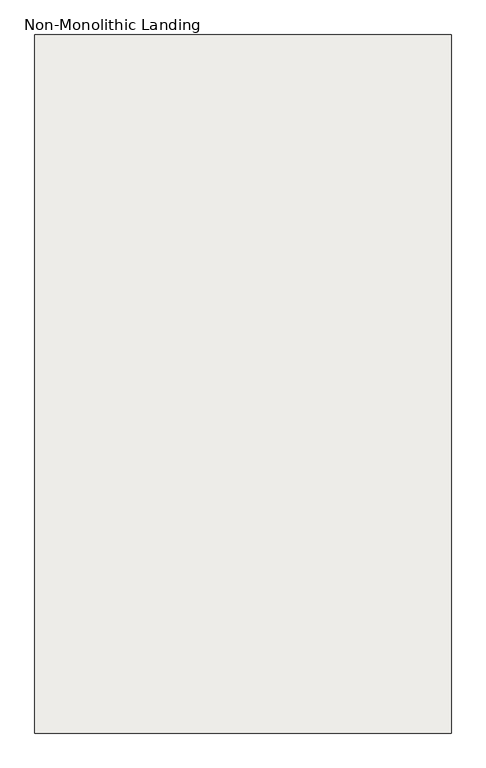
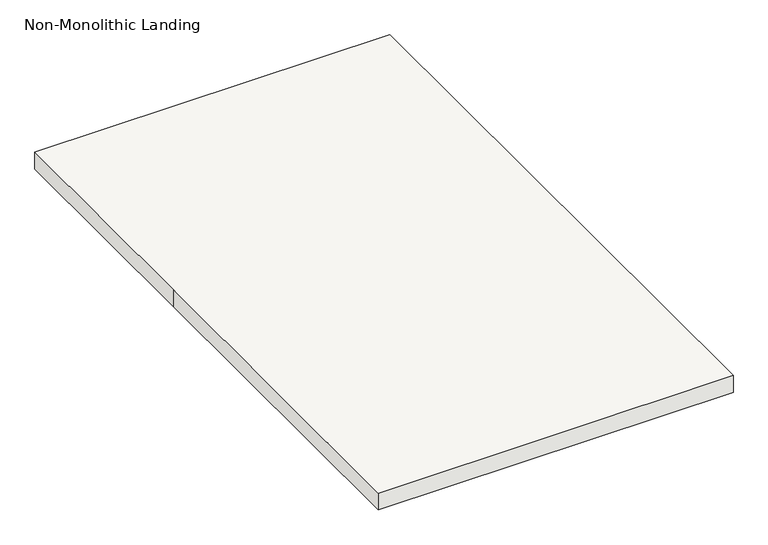
"""IFC4 building model written with IfcOpenShell, lengths in millimetres: slab geometry, Non-Monolithic Landing."""

import ifcopenshell
import ifcopenshell.guid

model = None  # the IFC model being written
_history = None  # IfcOwnerHistory: only IFC2X3 demands one
_inside = {}  # id of a spatial element -> (the spatial element, [elements in it])
_under = {}  # id of a project, library or spatial element -> (it, [spatial elements below it])
_declared = {}  # id of a project -> (the project, [libraries it declares])
_typed = {}  # id of a type object -> (the type object, [elements of that type])
_made_of = {}  # id of a material, layer set ... -> (it, [elements and type objects made of it])


def new_model(schema):
    """Start an empty IFC model of exactly this schema.

    Asked for "IFC4X3", IfcOpenShell would pick the latest addendum, in which some entities
    have other attributes; the version numbers below select the first issue.
    IFC2X3 requires an IfcOwnerHistory on every rooted entity: one is made here for all.
    """
    global model, _history
    if schema == "IFC4X3":
        model = ifcopenshell.file(schema_version=(4, 3, 0, 0))
    else:
        model = ifcopenshell.file(schema=schema)
    _inside.clear()
    _under.clear()
    _declared.clear()
    _typed.clear()
    _made_of.clear()
    _history = None
    if model.schema == "IFC2X3":
        org = make("IfcOrganization", Name="unknown")
        user = make(
            "IfcPersonAndOrganization",
            ThePerson=make("IfcPerson", FamilyName="unknown"),
            TheOrganization=org,
        )
        app = make(
            "IfcApplication",
            ApplicationDeveloper=org,
            Version="unknown",
            ApplicationFullName="unknown",
            ApplicationIdentifier="unknown",
        )
        _history = make(
            "IfcOwnerHistory",
            OwningUser=user,
            OwningApplication=app,
            ChangeAction="ADDED",
            CreationDate=0,
        )
    return model


def make(cls, **values):
    """One entity of the class cls with the attributes given. An attribute that is None is left unset."""
    return model.create_entity(
        cls, **{name: value for name, value in values.items() if value is not None}
    )


def rooted(cls, **values):
    """An entity with a GlobalId (a new one), such as an element, a storey or a relation."""
    return make(cls, GlobalId=ifcopenshell.guid.new(), OwnerHistory=_history, **values)


def si_unit(unit_type, name, prefix=None):
    """IfcSIUnit, for example si_unit("LENGTHUNIT", "METRE", prefix="MILLI")."""
    return make("IfcSIUnit", UnitType=unit_type, Prefix=prefix, Name=name)


def assignment(units):
    """IfcUnitAssignment: the units of a project."""
    return None if units is None else make("IfcUnitAssignment", Units=units)


def point(xyz):
    """IfcCartesianPoint."""
    return None if xyz is None else make("IfcCartesianPoint", Coordinates=xyz)


def direction(xyz):
    """IfcDirection."""
    return None if xyz is None else make("IfcDirection", DirectionRatios=xyz)


def frame(location, z_axis=None, x_axis=None):
    """IfcAxis2Placement3D, a coordinate frame: its origin and axes. An axis left out is left unset."""
    return make(
        "IfcAxis2Placement3D",
        Location=point(location),
        Axis=direction(z_axis),
        RefDirection=direction(x_axis),
    )


def origin():
    """The frame at (0, 0, 0) with its axes left unset."""
    return frame((0.0, 0.0, 0.0))


def place(relative_to, where):
    """IfcLocalPlacement: puts the frame where relative to a parent placement (None: the world)."""
    return make(
        "IfcLocalPlacement", PlacementRelTo=relative_to, RelativePlacement=where
    )


def context(
    kind, dimensions, precision=None, world=None, true_north=None, identifier=None
):
    """IfcGeometricRepresentationContext, for example the 3D "Model" context."""
    return make(
        "IfcGeometricRepresentationContext",
        ContextIdentifier=identifier,
        ContextType=kind,
        CoordinateSpaceDimension=dimensions,
        Precision=precision,
        WorldCoordinateSystem=world,
        TrueNorth=true_north,
    )


def project(units=None, contexts=None):
    """IfcProject with its units and contexts."""
    return rooted(
        "IfcProject",
        Name="project",
        RepresentationContexts=contexts,
        UnitsInContext=assignment(units),
    )


def spatial(cls, under=None, at=None, **own):
    """A site, building, storey or space (cls), placed at a placement, below another one or the project."""
    s = rooted(cls, ObjectPlacement=at, **own)
    if under is not None:
        _under.setdefault(under.id(), (under, []))[1].append(s)
    return s


def polyline(points):
    """IfcPolyline through the points."""
    return make("IfcPolyline", Points=[point(p) for p in points])


def outline(outer, holes=None, kind="AREA"):
    """IfcArbitraryClosedProfileDef: a profile drawn as a closed curve; with holes, ...WithVoids."""
    if holes is None:
        return make("IfcArbitraryClosedProfileDef", ProfileType=kind, OuterCurve=outer)
    return make(
        "IfcArbitraryProfileDefWithVoids",
        ProfileType=kind,
        OuterCurve=outer,
        InnerCurves=holes,
    )


def extrude(swept, where, along, depth):
    """IfcExtrudedAreaSolid: the profile swept, set in the frame where, extruded along a direction by depth."""
    return make(
        "IfcExtrudedAreaSolid",
        SweptArea=swept,
        Position=where,
        ExtrudedDirection=direction(along),
        Depth=depth,
    )


def shape(context_of_items, identifier, shape_type, items):
    """IfcShapeRepresentation: the items that make up one representation, for example the "Body"."""
    return make(
        "IfcShapeRepresentation",
        ContextOfItems=context_of_items,
        RepresentationIdentifier=identifier,
        RepresentationType=shape_type,
        Items=items,
    )


def source(mapping_origin, context_of_items, identifier, shape_type, items):
    """IfcRepresentationMap: a shape defined once, which mapped items show again and again."""
    return make(
        "IfcRepresentationMap",
        MappingOrigin=mapping_origin,
        MappedRepresentation=shape(context_of_items, identifier, shape_type, items),
    )


def transform(
    local_origin,
    x_axis=None,
    y_axis=None,
    z_axis=None,
    scale=None,
    scale2=None,
    scale3=None,
    uniform=True,
):
    """IfcCartesianTransformationOperator3D, or its non-uniform kind. x_axis, y_axis, z_axis: its Axis1, 2, 3."""
    if uniform:
        return make(
            "IfcCartesianTransformationOperator3D",
            Axis1=direction(x_axis),
            Axis2=direction(y_axis),
            LocalOrigin=point(local_origin),
            Scale=scale,
            Axis3=direction(z_axis),
        )
    return make(
        "IfcCartesianTransformationOperator3DnonUniform",
        Axis1=direction(x_axis),
        Axis2=direction(y_axis),
        LocalOrigin=point(local_origin),
        Scale=scale,
        Axis3=direction(z_axis),
        Scale2=scale2,
        Scale3=scale3,
    )


def mapped(mapping_source, mapping_target):
    """IfcMappedItem: shows the shape of a source again, moved by a transform."""
    return make(
        "IfcMappedItem", MappingSource=mapping_source, MappingTarget=mapping_target
    )


def made_of(thing, what):
    """Note that an element or type object is made of a material, layer set ...; save() writes the relation."""
    if what is not None:
        _made_of.setdefault(what.id(), (what, []))[1].append(thing)
    return thing


def element(
    cls,
    number,
    at=None,
    inside=None,
    cuts=None,
    type_object=None,
    material=None,
    context=None,
    identifier="Body",
    shape_type=None,
    held_by="IfcProductDefinitionShape",
    body=None,
    shapes=None,
    **own,
):
    """One element of the class cls, such as IfcWall. Its Tag is "e" and its number.

    at: its placement. inside: the storey or other place that contains it. cuts: it is an
    opening in that element (IfcRelVoidsElement). A single representation is given by context,
    identifier, shape_type and body (its items); several are given by shapes. held_by: the class
    of the entity that holds the representations. save() writes the other relations.
    """
    e = rooted(cls, Tag="e%d" % number, ObjectPlacement=at, **own)
    if body is not None:
        shapes = [shape(context, identifier, shape_type, body)]
    if shapes is not None:
        e.Representation = make(held_by, Representations=shapes)
    if inside is not None:
        _inside.setdefault(inside.id(), (inside, []))[1].append(e)
    if cuts is not None:
        rooted(
            "IfcRelVoidsElement", RelatingBuildingElement=cuts, RelatedOpeningElement=e
        )
    if type_object is not None:
        _typed.setdefault(type_object.id(), (type_object, []))[1].append(e)
    return made_of(e, material)


def aggregate(whole, parts):
    """IfcRelAggregates: a whole, such as a stair, and the parts it consists of."""
    return rooted("IfcRelAggregates", RelatingObject=whole, RelatedObjects=parts)


def save(model, path):
    """Write the relations noted so far, then the file.

    IfcRelAggregates (storeys below a building ...), IfcRelContainedInSpatialStructure (elements
    in a storey), IfcRelDefinesByType, IfcRelAssociatesMaterial and IfcRelDeclares: one each for
    every whole, place, type object, material and project.
    """
    for whole, parts in _under.values():
        aggregate(whole, parts)
    for where, things in _inside.values():
        rooted(
            "IfcRelContainedInSpatialStructure",
            RelatedElements=things,
            RelatingStructure=where,
        )
    for kind, things in _typed.values():
        rooted("IfcRelDefinesByType", RelatedObjects=things, RelatingType=kind)
    for what, things in _made_of.values():
        rooted("IfcRelAssociatesMaterial", RelatedObjects=things, RelatingMaterial=what)
    for by, libraries in _declared.values():
        rooted("IfcRelDeclares", RelatingContext=by, RelatedDefinitions=libraries)
    model.write(path)


def non_monolithic_landing_a6d5fe41(model_context):
    return source(origin(), model_context, "Body", "SweptSolid", [
        extrude(outline(polyline([(21529.836337, -3576.2808257), (21529.836337, -2900.524372), (22529.836337, -2900.524372), (22529.836337, -4576.2808257), (21529.836337, -4576.2808257), (21529.836337, -3576.2808257)])), frame((0.0, 0.0, 1859.0909091), z_axis=(0.0, 0.0, 1.0), x_axis=(1.0, 0.0, 0.0)), (0.0, 0.0, 1.0), 50.0),
    ])


if __name__ == "__main__":
    model = new_model("IFC4")
    model_context = context("Model", 3, world=origin())
    ifc_project = project(units=[si_unit("LENGTHUNIT", "METRE", prefix="MILLI")], contexts=[model_context])
    site = spatial("IfcSite", under=ifc_project)
    building = spatial("IfcBuilding", under=site)
    placement = place(None, origin())
    non_monolithic_landing_shape = non_monolithic_landing_a6d5fe41(model_context)
    element("IfcSlab", 1, ObjectType="Non-Monolithic Landing", at=placement, inside=building, context=model_context, shape_type="MappedRepresentation", body=[
        mapped(non_monolithic_landing_shape, transform((0.0, 0.0, 0.0), x_axis=(1.0, 0.0, 0.0), y_axis=(0.0, 1.0, 0.0), z_axis=(0.0, 0.0, 1.0))),
    ])
    save(model, "model.ifc")
